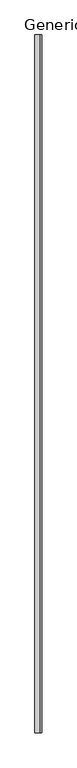
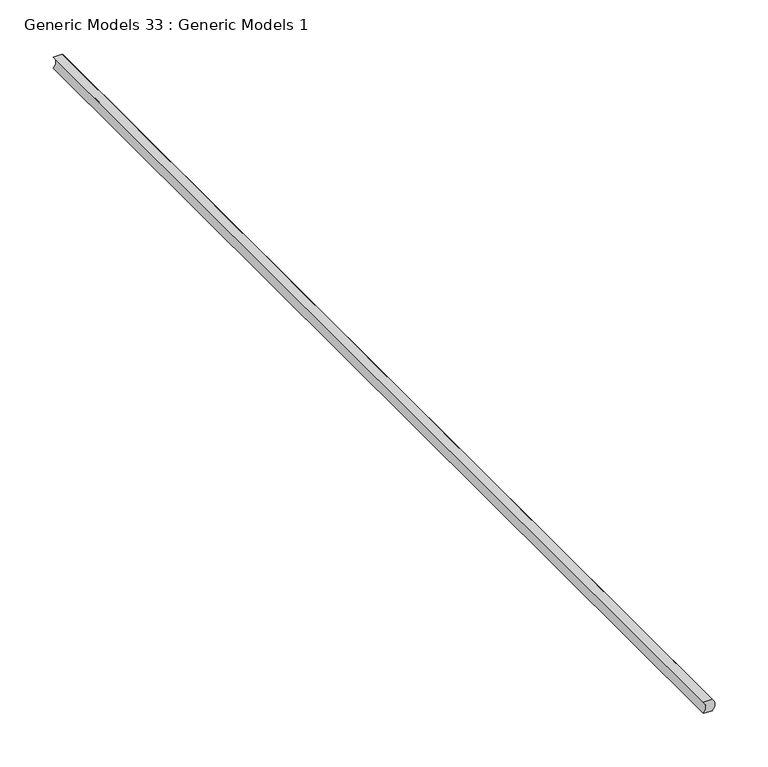
"""IFC4 building model written with IfcOpenShell, lengths in millimetres: proxy geometry, Generic Models 33 : Generic Models 1."""

from ifc_helpers import new_model, si_unit, point, frame, frame_2d, origin, place, context, project, spatial, polyline, circle_curve, trimmed, segment, composite_curve, outline, extrude, source, transform, mapped, element, save


def generic_models_33_generic_models_1_37963aa5(model_context):
    return source(origin(), model_context, "Body", "SweptSolid", [
        extrude(outline(composite_curve([segment(polyline([(520.3026794, 52542.4946108), (520.3026794, 52552.0196108)]), True, "CONTINUOUS"), segment(trimmed(circle_curve(frame_2d((526.6526794, 52546.1901298)), 8.620055), [point((520.3026794, 52552.0196108))], [point((533.0026794, 52552.0196108))], False, "CARTESIAN"), True, "CONTINUOUS"), segment(polyline([(533.0026794, 52552.0196108), (533.0026794, 52542.4946108)]), True, "CONTINUOUS"), segment(trimmed(circle_curve(frame_2d((526.6526794, 52536.6651298)), 8.620055), [point((533.0026794, 52542.4946108))], [point((520.3026794, 52542.4946108))], True, "CARTESIAN"), True, "CONTINUOUS")], self_intersect=False)), frame((0.0, 0.0, 0.0), z_axis=(0.0, 1.0, 0.0), x_axis=(0.0, 0.0, 1.0)), (0.0, 0.0, 1.0), 1219.2),
    ])


if __name__ == "__main__":
    model = new_model("IFC4")
    model_context = context("Model", 3, world=origin())
    ifc_project = project(units=[si_unit("LENGTHUNIT", "METRE", prefix="MILLI")], contexts=[model_context])
    site = spatial("IfcSite", under=ifc_project)
    building = spatial("IfcBuilding", under=site)
    placement = place(None, origin())
    generic_models_33_generic_models_1_shape = generic_models_33_generic_models_1_37963aa5(model_context)
    element("IfcBuildingElementProxy", 1, Name="Generic Models 33 : Generic Models 1", ObjectType="Generic Models 33 : Generic Models 1", at=placement, inside=building, context=model_context, shape_type="MappedRepresentation", body=[
        mapped(generic_models_33_generic_models_1_shape, transform((0.0, 0.0, 0.0), x_axis=(1.0, 0.0, 0.0), y_axis=(0.0, 1.0, 0.0), z_axis=(0.0, 0.0, 1.0))),
    ])
    save(model, "model.ifc")

# Revit data of these elements
# Element 1 (IfcBuildingElementProxy, "Generic Models 33 : Generic Models 1")
#   Materials on its faces: "ACOUSTICAL SEALANT"
# Materials
#   "ACOUSTICAL SEALANT": class "Unassigned", colour RGB 120 120 120, transparency 0, Cost = 0
